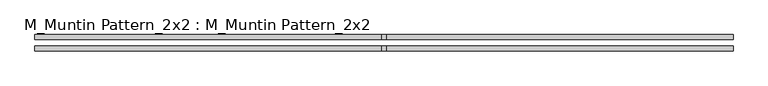
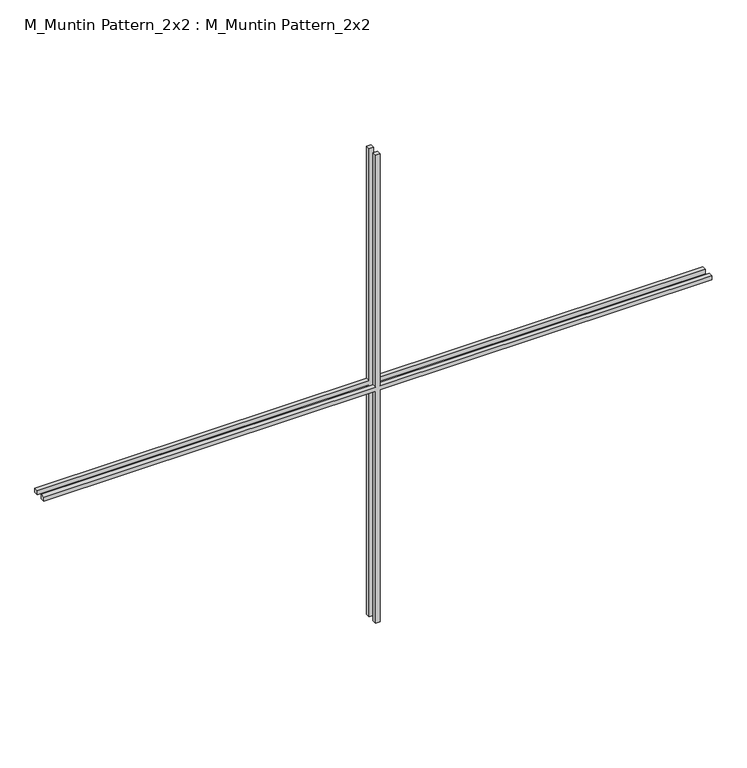
"""IFC4 building model written with IfcOpenShell, lengths in millimetres: proxy geometry, M_Muntin Pattern_2x2 : M_Muntin Pattern_2x2."""

from ifc_helpers import new_model, si_unit, frame, origin, place, context, project, spatial, polyline, outline, extrude, source, transform, mapped, element, save


def m_muntin_pattern_2x2_m_muntin_pattern_2x2_aeef4309(model_context):
    return source(origin(), model_context, "Body", "SweptSolid", [
        extrude(outline(polyline([(718.25, -6.35), (718.25, -961.9), (705.55, -961.9), (705.55, -6.35), (0.0, -6.35), (0.0, 6.35), (705.55, 6.35), (705.55, 961.9), (718.25, 961.9), (718.25, 6.35), (1423.8, 6.35), (1423.8, -6.35), (718.25, -6.35)])), frame((0.0, -22.225, 0.0), z_axis=(0.0, 1.0, 0.0), x_axis=(0.0, 0.0, 1.0)), (0.0, 0.0, 1.0), 12.7),
        extrude(outline(polyline([(718.25, -6.35), (718.25, -961.9), (705.55, -961.9), (705.55, -6.35), (0.0, -6.35), (0.0, 6.35), (705.55, 6.35), (705.55, 961.9), (718.25, 961.9), (718.25, 6.35), (1423.8, 6.35), (1423.8, -6.35), (718.25, -6.35)])), frame((0.0, 9.525, 0.0), z_axis=(0.0, 1.0, 0.0), x_axis=(0.0, 0.0, 1.0)), (0.0, 0.0, 1.0), 12.7),
    ])


if __name__ == "__main__":
    model = new_model("IFC4")
    model_context = context("Model", 3, world=origin())
    ifc_project = project(units=[si_unit("LENGTHUNIT", "METRE", prefix="MILLI")], contexts=[model_context])
    site = spatial("IfcSite", under=ifc_project)
    building = spatial("IfcBuilding", under=site)
    placement = place(None, origin())
    m_muntin_pattern_2x2_m_muntin_pattern_2x2_shape = m_muntin_pattern_2x2_m_muntin_pattern_2x2_aeef4309(model_context)
    element("IfcBuildingElementProxy", 1, Name="M_Muntin Pattern_2x2 : M_Muntin Pattern_2x2", ObjectType="M_Muntin Pattern_2x2 : M_Muntin Pattern_2x2", at=placement, inside=building, context=model_context, shape_type="MappedRepresentation", body=[
        mapped(m_muntin_pattern_2x2_m_muntin_pattern_2x2_shape, transform((0.0, 0.0, 0.0), x_axis=(1.0, 0.0, 0.0), y_axis=(0.0, 1.0, 0.0), z_axis=(0.0, 0.0, 1.0))),
    ])
    save(model, "model.ifc")

# Revit data of these elements
# Type "M_Muntin Pattern_2x2 : M_Muntin Pattern_2x2"
#   Width [instance default] = 1200 mm
#   Thickness = 12.7 mm
#   Height [instance default] = 1200 mm
#   Distance = 19.05 mm
#   Interior Material [instance default] = none
#   Exterior Material [instance default] = none
#   Default Elevation = 0
# Element 1 (IfcBuildingElementProxy, "M_Muntin Pattern_2x2 : M_Muntin Pattern_2x2")
#   Width = 1923.8 mm
#   Height = 1423.8 mm
#   Interior Material = Wood - Stained
#   Exterior Material = Clad - White
#   Materials on its faces: "Clad - White", "Wood - Stained"
# Materials
#   "Clad - White": class "Wood", colour RGB 245 245 243, transparency 0, Cost = 0
#   "Wood - Stained": class "Wood", colour RGB 173 132 96, transparency 0, Cost = 0
